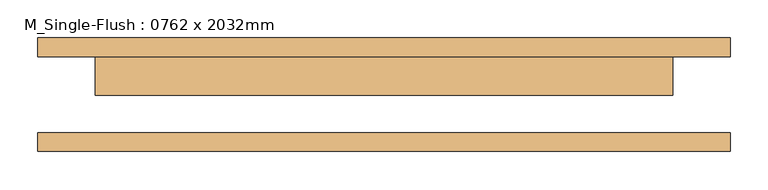
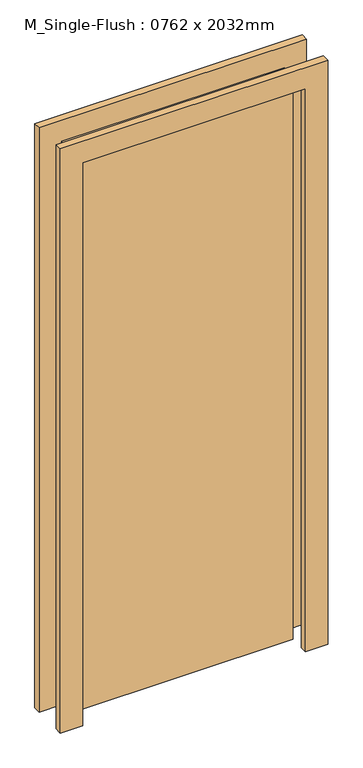
"""IFC4 building model written with IfcOpenShell, lengths in millimetres: door geometry, M_Single-Flush : 0762 x 2032mm."""

from ifc_helpers import new_model, si_unit, frame, origin, origin_with_axes, place, context, project, spatial, polyline, outline, extrude, source, transform, mapped, element, save


def m_single_flush_0762_x_2032mm_6732b1f7(model_context):
    return source(origin(), model_context, "Body", "SweptSolid", [
        extrude(outline(polyline([(2108.0, -457.0), (0.0, -457.0), (0.0, -381.0), (2032.0, -381.0), (2032.0, 381.0), (0.0, 381.0), (0.0, 457.0), (2108.0, 457.0), (2108.0, -457.0)])), frame((0.0, 50.0, 0.0), z_axis=(0.0, 1.0, 0.0), x_axis=(0.0, 0.0, 1.0)), (0.0, 0.0, 1.0), 25.0),
        extrude(outline(polyline([(2108.0, 457.0), (2108.0, -457.0), (0.0, -457.0), (0.0, -381.0), (2032.0, -381.0), (2032.0, 381.0), (0.0, 381.0), (0.0, 457.0), (2108.0, 457.0)])), frame((0.0, -75.0, 0.0), z_axis=(0.0, 1.0, 0.0), x_axis=(0.0, 0.0, 1.0)), (0.0, 0.0, 1.0), 25.0),
        extrude(outline(polyline([(381.0, -1.0), (-381.0, -1.0), (-381.0, 50.0), (381.0, 50.0), (381.0, -1.0)])), origin_with_axes(), (0.0, 0.0, 1.0), 2032.0),
    ])


if __name__ == "__main__":
    model = new_model("IFC4")
    model_context = context("Model", 3, world=origin())
    ifc_project = project(units=[si_unit("LENGTHUNIT", "METRE", prefix="MILLI")], contexts=[model_context])
    site = spatial("IfcSite", under=ifc_project)
    building = spatial("IfcBuilding", under=site)
    placement = place(None, origin())
    m_single_flush_0762_x_2032mm_shape = m_single_flush_0762_x_2032mm_6732b1f7(model_context)
    element("IfcDoor", 1, ObjectType="M_Single-Flush : 0762 x 2032mm", at=placement, inside=building, context=model_context, shape_type="MappedRepresentation", body=[
        mapped(m_single_flush_0762_x_2032mm_shape, transform((0.0, 0.0, 0.0), x_axis=(1.0, 0.0, 0.0), y_axis=(0.0, 1.0, 0.0), z_axis=(0.0, 0.0, 1.0))),
    ])
    save(model, "model.ifc")

# Revit data of these elements
# Type "M_Single-Flush : 0762 x 2032mm"
#   Type Mark = "19"
#   Thickness = 0.051 m
#   Height = 2.032 m
#   Trim Projection Ext = 0.025 m
#   Trim Projection Int = 0.025 m
#   Trim Width = 0.076 m
#   Width = 0.762 m
#   Door Material = Door - Panel
#   Frame Material = Door - Frame
#   Function = (empty or 0)
#   Wall Closure = (empty or 0)
# Element 1 (IfcDoor, "M_Single-Flush : 0762 x 2032mm")
#   Materials on its faces: "Door - Frame", "Door - Panel"
# Materials
#   "Door - Panel": class "Wood", colour RGB 114 82 51, transparency 0
#   "Door - Frame": class "Miscellaneous", colour RGB 153 76 43, transparency 0
